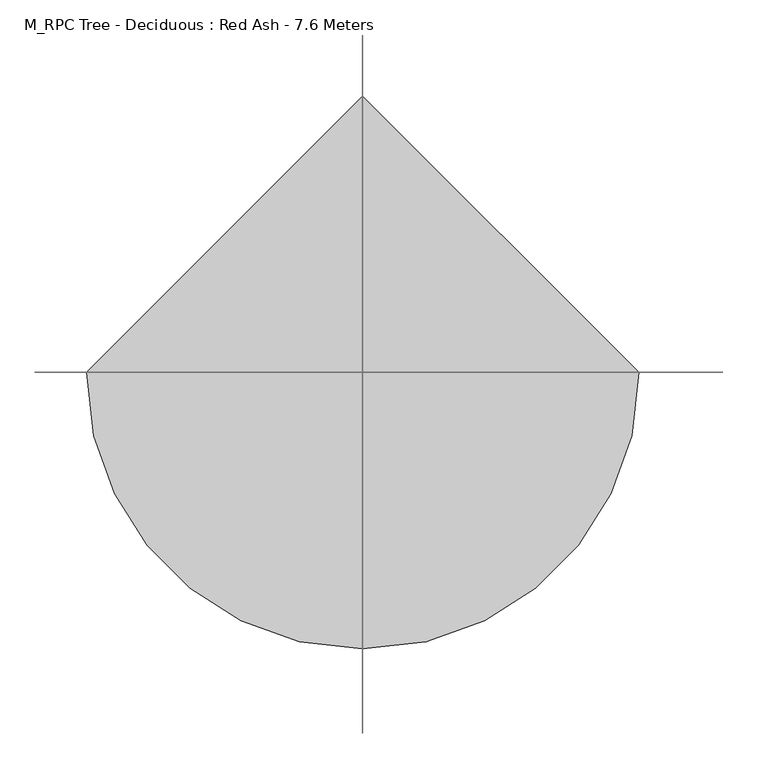
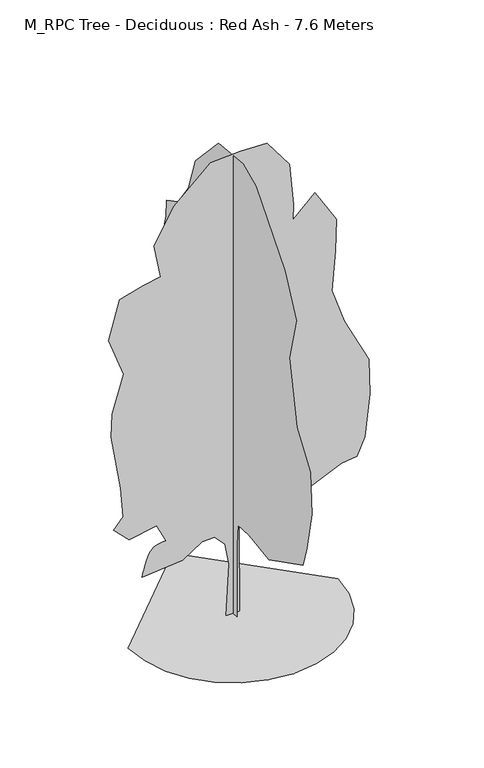
"""IFC4 building model written with IfcOpenShell, lengths in millimetres: geographic element geometry, M_RPC Tree - Deciduous : Red Ash - 7.6 Meters."""

from ifc_helpers import new_model, si_unit, origin, place, context, project, spatial, triangles, source, transform, mapped, element, save


def m_rpc_tree_deciduous_red_ash_7_6_meters_40acba24(model_context):
    return source(origin(), model_context, "Body", "Tessellation", [
        triangles([(-1640.6350319, 0.0, 6.17e-05), (-1597.2618073, -375.9250917, 6.17e-05), (-1473.7362076, -721.1521299, 6.17e-05), (-1279.9481815, -1025.7899305, 6.17e-05), (-1025.7900759, -1279.9483269, 6.17e-05), (-721.1519119, -1473.7357716, 6.17e-05), (-375.9249101, -1597.2618073, 6.17e-05), (7.17e-05, -1640.6350319, 6.17e-05), (375.9250917, -1597.2619526, 6.17e-05), (721.1521299, -1473.7360622, 6.17e-05), (1025.7900759, -1279.9481815, 6.17e-05), (1279.9486176, -1025.7900759, 6.17e-05), (1473.7359169, -721.1519119, 6.17e-05), (1597.2618073, -375.9248374, 6.17e-05), (1640.6350319, 0.0001434, 6.17e-05), (-0.0002151, 1640.6350319, 6.17e-05), (-1.07e-05, -102.5763152, 0.0), (2.5e-05, -100.9809819, 1191.4187742), (3.22e-05, -129.5410573, 1533.7667004), (7e-07, -437.6736119, 1554.0757805), (-5.76e-05, -973.8285673, 1474.4268631), (-0.0001401, -1898.6961697, 1943.5624718), (-0.0001409, -2005.9272697, 2292.063438), (-0.0001357, -2139.9660358, 2935.4496025), (-0.0001116, -2099.7546822, 3605.6435783), (-5.8e-05, -1735.814106, 4130.1484818), (-5.5e-06, -1523.3897175, 5147.0898972), (-3.5e-06, -1711.0423622, 5870.899205), (4.78e-05, -1402.7536217, 6514.2855148), (0.0001565, -625.3287638, 7439.1534805), (0.000198, -272.4836404, 7598.1990051), (0.0002655, 393.3664327, 7532.9808929), (0.0003113, 1023.3488731, 6862.7869171), (0.0003141, 1211.0034073, 6299.8236053), (0.0003314, 1492.4837551, 5897.7074524), (0.0003588, 1800.7742397, 5736.8608749), (0.0003522, 1814.1780727, 5468.7830521), (0.0003514, 1894.6015068, 5160.4937302), (0.0003267, 1760.5627407, 4798.5893669), (0.0003288, 1881.1976738, 4450.088546), (0.000327, 2001.8324615, 3967.5488136), (0.0003203, 1975.0247955, 3833.5096115), (0.0002869, 1747.159053, 3511.8164566), (0.0002722, 1732.7516476, 3069.4885139), (0.0002625, 1720.3510963, 2788.0068581), (0.0002535, 1733.7549294, 2439.5063278), (0.0002406, 1747.159053, 1956.9668861), (0.0002166, 1559.5046642, 1809.523851), (0.0001802, 1211.0038433, 1809.523851), (0.0001822, 1371.8504208, 1313.580431), (0.0001711, 1344.9556961, 1032.1683203), (0.0001512, 1100.1359739, 1224.6137684), (9.84e-05, 627.810589, 1103.8028286), (9.77e-05, 550.2637599, 1353.49907), (6.27e-05, 215.346067, 1350.4488201), (5.01e-05, 130.4579254, 1225.1105404), (3.26e-05, 79.3405423, 816.1354311), (1.17e-05, 111.8716144, 1.28e-05), (-110.5798692, 4.8e-06, 4.45e-05), (-66.5363775, -9.62e-05, 831.3140104), (-128.9679092, -0.0001356, 1184.825572), (-290.0246482, -0.0001497, 1361.7341778), (-482.3670685, -0.0001405, 1355.1302204), (-794.1779051, -0.0001027, 1152.7338535), (-1424.1603092, -6.88e-05, 1099.1184488), (-1415.4458702, -7.33e-05, 1133.781086), (-1406.1451298, -7.8e-05, 1169.6158899), (-1395.6722225, -8.3e-05, 1207.7952456), (-1383.4407017, -8.85e-05, 1249.4921917), (-1368.8645565, -9.46e-05, 1295.8774418), (-1351.3574856, -0.0001016, 1348.1257061), (-1330.3333328, -0.0001096, 1407.4074074), (-1303.8382931, -0.0001173, 1462.3908245), (-1271.0123898, -0.0001236, 1502.6024689), (-1232.9109364, -0.0001286, 1530.5039635), (-1190.588883, -0.0001326, 1548.5586754), (-1145.1018339, -0.0001358, 1559.2267742), (-1097.5041578, -0.0001386, 1564.971191), (-1048.8515316, -0.0001411, 1568.2539848), (-1196.294058, -0.0001698, 1863.1393284), (-1625.218531, -0.0001415, 1782.7160397), (-1866.4879612, -0.0001597, 2023.9863419), (-1719.0452168, -0.0001869, 2198.236607), (-1759.2568611, -0.0002427, 2680.7764847), (-1906.6994602, -0.0003433, 3578.8359123), (-1893.4979404, -0.0003882, 3950.7687332), (-1715.4032879, -0.0004676, 4551.3483536), (-1946.9112499, -0.0005333, 5187.3013962), (-1772.6605488, -0.0006144, 5803.88004), (-1410.7561855, -0.000643, 5911.1112854), (-1135.4252443, -0.0006608, 5959.6792511), (-1236.5059204, -0.0007209, 6500.8816818), (-928.2163805, -0.0007999, 7050.4411606), (-351.8493811, -0.0008874, 7573.192392), (117.2860368, -0.0009111, 7600.000058), (532.8066133, -0.0009277, 7586.5956436), (881.3074705, -0.000887, 7117.4603256), (945.3842279, -0.0008079, 6430.5952744), (936.1832634, -0.0007775, 6178.7100677), (1283.4236961, -0.0008311, 6500.8816818), (1618.5208294, -0.0007802, 5951.3222031), (1605.1169964, -0.0007177, 5432.2143539), (1545.3907001, -0.0006383, 4788.0519287), (1739.1557625, -0.0005793, 4222.2222221), (2126.1689129, -0.0005054, 3460.0925789), (2138.5076946, -0.0004374, 2885.2169128), (2060.848772, -0.0003521, 2198.2364616), (1940.213839, -0.0003133, 1916.7548058), (1698.9439728, -0.0002996, 1889.9471397), (1229.8082188, -0.0002535, 1675.4849396), (814.2876514, -0.0002002, 1380.5997414), (256.8007496, -0.0002044, 1620.3048775), (92.8066444, -0.0001762, 1443.8352711), (103.8818677, -4.5e-06, 3.51e-05)], [[15, 16, 1], [14, 15, 1], [14, 1, 2], [13, 14, 2], [13, 2, 3], [13, 3, 4], [12, 13, 4], [11, 12, 4], [11, 4, 5], [11, 5, 6], [11, 6, 7], [11, 7, 8], [11, 8, 9], [11, 9, 10], [50, 51, 52], [57, 58, 17], [57, 17, 18], [56, 57, 18], [56, 18, 19], [55, 56, 19], [49, 50, 52], [52, 53, 54], [49, 52, 54], [35, 36, 37], [46, 47, 48], [46, 48, 49], [21, 22, 23], [20, 21, 23], [20, 23, 24], [20, 24, 25], [20, 25, 26], [19, 20, 26], [19, 26, 27], [45, 46, 49], [31, 32, 33], [30, 31, 33], [29, 30, 33], [29, 33, 34], [28, 29, 34], [27, 28, 34], [19, 27, 34], [19, 34, 35], [19, 35, 37], [19, 37, 38], [19, 38, 39], [19, 39, 40], [19, 40, 41], [19, 41, 42], [19, 42, 43], [19, 43, 44], [19, 44, 45], [19, 45, 49], [19, 49, 54], [55, 19, 54], [64, 65, 66], [64, 66, 67], [64, 67, 68], [99, 100, 101], [64, 68, 69], [64, 69, 70], [64, 70, 71], [114, 59, 60], [113, 114, 60], [113, 60, 61], [113, 61, 62], [64, 71, 72], [64, 72, 73], [64, 73, 74], [64, 74, 75], [64, 75, 76], [64, 76, 77], [64, 77, 78], [64, 78, 79], [63, 64, 79], [81, 82, 83], [80, 81, 83], [99, 101, 102], [107, 108, 109], [110, 111, 112], [88, 89, 90], [87, 88, 90], [87, 90, 91], [80, 83, 84], [95, 96, 97], [95, 97, 98], [94, 95, 98], [93, 94, 98], [92, 93, 98], [91, 92, 98], [91, 98, 99], [87, 91, 99], [87, 99, 102], [87, 102, 103], [87, 103, 104], [86, 87, 104], [85, 86, 104], [84, 85, 104], [80, 84, 104], [80, 104, 105], [80, 105, 106], [80, 106, 107], [80, 107, 109], [80, 109, 110], [80, 110, 112], [79, 80, 112], [63, 79, 112], [62, 63, 112], [113, 62, 112]], closed=False),
    ])


if __name__ == "__main__":
    model = new_model("IFC4")
    model_context = context("Model", 3, world=origin())
    ifc_project = project(units=[si_unit("LENGTHUNIT", "METRE", prefix="MILLI")], contexts=[model_context])
    site = spatial("IfcSite", under=ifc_project)
    building = spatial("IfcBuilding", under=site)
    placement = place(None, origin())
    m_rpc_tree_deciduous_red_ash_7_6_meters_shape = m_rpc_tree_deciduous_red_ash_7_6_meters_40acba24(model_context)
    element("IfcGeographicElement", 1, ObjectType="M_RPC Tree - Deciduous : Red Ash - 7.6 Meters", at=placement, inside=building, context=model_context, shape_type="MappedRepresentation", body=[
        mapped(m_rpc_tree_deciduous_red_ash_7_6_meters_shape, transform((0.0, 0.0, 0.0), x_axis=(1.0, 0.0, 0.0), y_axis=(0.0, 1.0, 0.0), z_axis=(0.0, 0.0, 1.0))),
    ])
    save(model, "model.ifc")

# Revit data of these elements
# Type "M_RPC Tree - Deciduous : Red Ash - 7.6 Meters"
#   built-in parameter 1005198 = "{2, 15},{22, RPC-8-G3GR-497X-PHW5-6},{1, 0},{1, 0},{2, 15},{1, 8},{5, Color},{1, 0},{1, 0},{3, 0.8},{3, 0.8},{3, 0.8},{1, 8},{7, BBoxMin},{1, 0},{1, 0},{1, 0},{1, 0},{1, 0},{1, 8},{7, BBoxMax},{1, 0},{1, 0},{1, 0},{1, 0},{1, 0},{2, 11},{9, RPCTypeId},{1, 0},{1, 0},{22, RPC-8-G3GR-497X-PHW5-6},{1, 6},{14, RPCPlantHeight},{1, 0},{1, 0},{7, 24.9344},{2, 11},{7, keyword},{1, 0},{1, 0},{34, :RPCs:Trees [General]:Geometry:RPC},{2, 11},{8, category},{1, 0},{1, 0},{15, Trees [General]},{2, 11},{12, LocalizedUID},{1, 0},{1, 0},{7, Red Ash},{2, 14},{6, Height},{1, 0},{1, 0},{7, 24.9344},{1, 2},{16, Cast Reflections},{1, 0},{1, 0},{1, 0},{1, 2},{6, Jitter},{1, 0},{1, 0},{1, 1},{1, 2},{9, Billboard},{1, 0},{1, 0},{1, 0},{1, 2},{12, Cast Shadows},{1, 0},{1, 0},{1, 1},{1, 2},{20, Apply Filter Effects},{1, 0},{1, 0},{1, 0},{2, 11},{28, Apply Filter Effects-Text-FC},{1, 0},{1, 0},{4, None},{21, assetlibrary_base.fbx},{1, 5},"
#   built-in parameter 1005195 = "RPC-8-G3GR-497X-PHW5-6"
#   Type Comments = "Red Ash"
#   Height = 7.600 m
#   Default Elevation = 0
